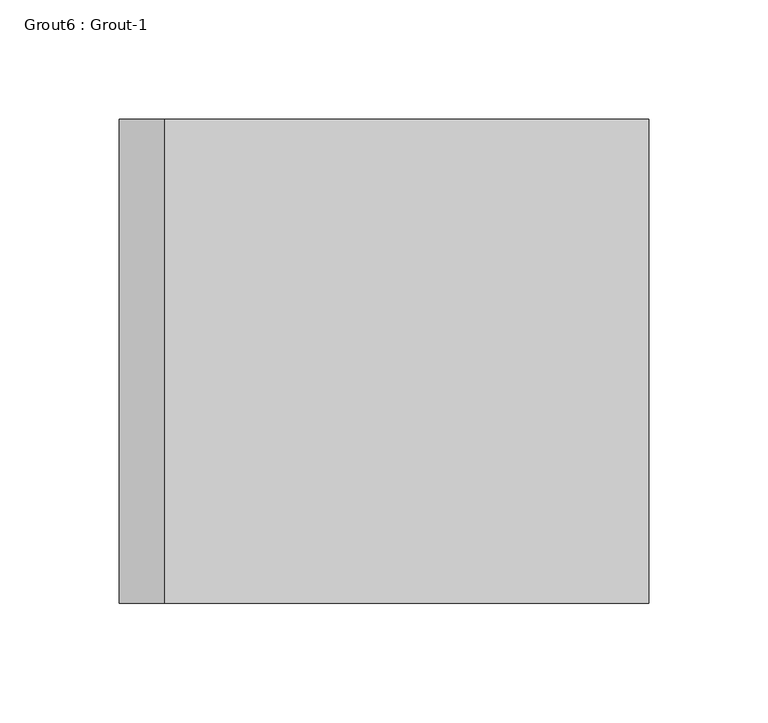
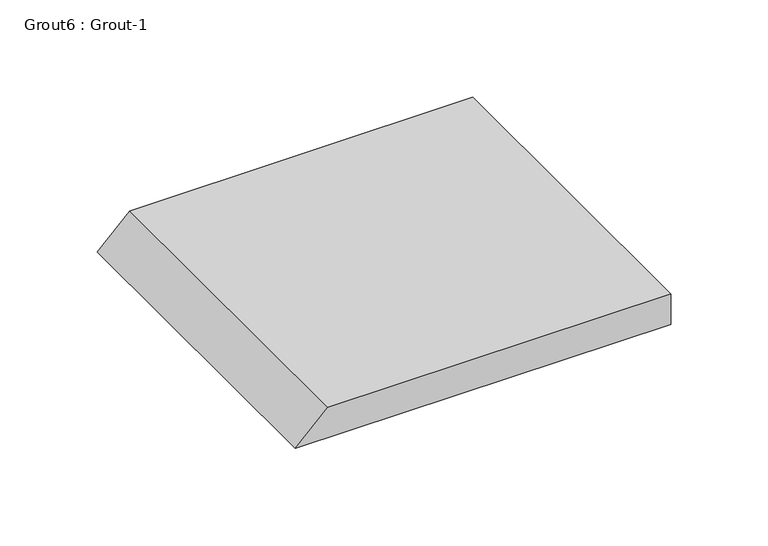
"""IFC4 building model written with IfcOpenShell, lengths in millimetres: proxy geometry, Grout6 : Grout-1."""

from ifc_helpers import new_model, si_unit, frame, origin, place, context, project, spatial, polyline, outline, extrude, source, transform, mapped, element, save


def grout6_grout_1_0f871906(model_context):
    return source(origin(), model_context, "Body", "SweptSolid", [
        extrude(outline(polyline([(19.05, 590115.4434739), (0.0, 590096.3934739), (0.0, 590318.6434739), (19.05, 590318.6434739), (19.05, 590115.4434739)])), frame((0.0, -535306.3413841, 0.0), z_axis=(0.0, 1.0, 0.0), x_axis=(0.0, 0.0, 1.0)), (0.0, 0.0, 1.0), 203.2),
    ])


if __name__ == "__main__":
    model = new_model("IFC4")
    model_context = context("Model", 3, world=origin())
    ifc_project = project(units=[si_unit("LENGTHUNIT", "METRE", prefix="MILLI")], contexts=[model_context])
    site = spatial("IfcSite", under=ifc_project)
    building = spatial("IfcBuilding", under=site)
    placement = place(None, origin())
    grout6_grout_1_shape = grout6_grout_1_0f871906(model_context)
    element("IfcBuildingElementProxy", 1, Name="Grout6 : Grout-1", ObjectType="Grout6 : Grout-1", at=placement, inside=building, context=model_context, shape_type="MappedRepresentation", body=[
        mapped(grout6_grout_1_shape, transform((0.0, 0.0, 0.0), x_axis=(1.0, 0.0, 0.0), y_axis=(0.0, 1.0, 0.0), z_axis=(0.0, 0.0, 1.0))),
    ])
    save(model, "model.ifc")

# Revit data of these elements
# Element 1 (IfcBuildingElementProxy, "Grout6 : Grout-1")
#   Materials on its faces: "3/4\" NON SHRINK GROUT"
# Materials
#   "3/4\" NON SHRINK GROUT": class "Generic", colour RGB 145 145 143, transparency 0, Cost = 0
